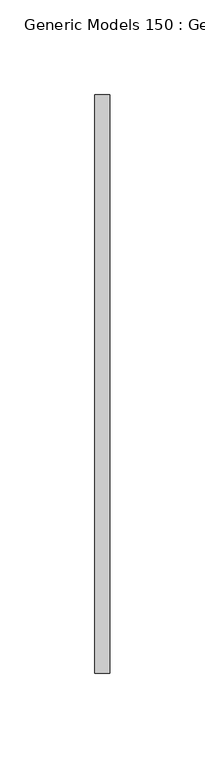
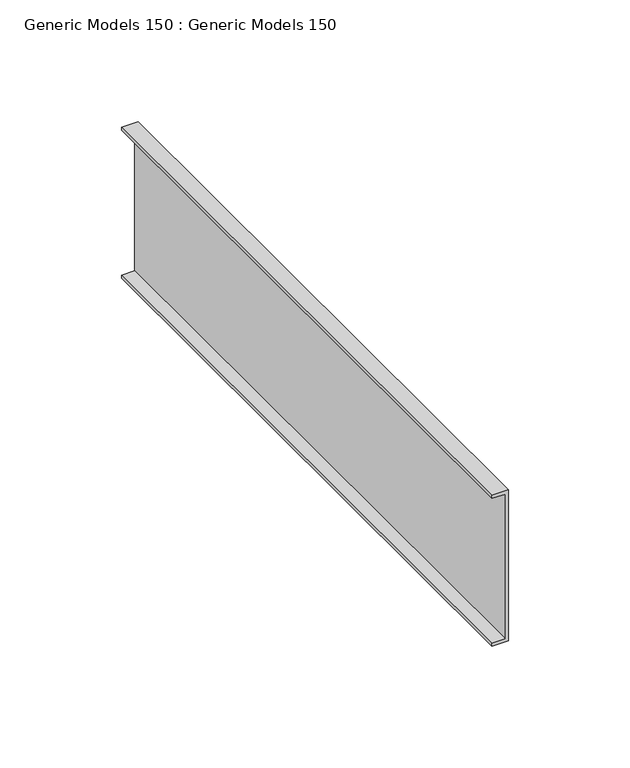
"""IFC4 building model written with IfcOpenShell, lengths in millimetres: proxy geometry, Generic Models 150 : Generic Models 150."""

from ifc_helpers import new_model, si_unit, frame, origin, place, context, project, spatial, polyline, outline, extrude, source, transform, mapped, element, save


def generic_models_150_generic_models_150_55fdb401(model_context):
    return source(origin(), model_context, "Body", "SweptSolid", [
        extrude(outline(polyline([(126267.7473366, 4973.2035579), (126195.0485482, 4973.2035579), (126195.0485482, 4966.8535579), (126193.4610482, 4966.8535579), (126193.4610482, 4974.7910579), (126269.3348366, 4974.7910579), (126269.3348366, 4966.8535579), (126267.7473366, 4966.8535579), (126267.7473366, 4973.2035579)])), frame((0.0, 399.7309662, 0.0), z_axis=(0.0, 1.0, 0.0), x_axis=(0.0, 0.0, 1.0)), (0.0, 0.0, 1.0), 304.8),
    ])


if __name__ == "__main__":
    model = new_model("IFC4")
    model_context = context("Model", 3, world=origin())
    ifc_project = project(units=[si_unit("LENGTHUNIT", "METRE", prefix="MILLI")], contexts=[model_context])
    site = spatial("IfcSite", under=ifc_project)
    building = spatial("IfcBuilding", under=site)
    placement = place(None, origin())
    generic_models_150_generic_models_150_shape = generic_models_150_generic_models_150_55fdb401(model_context)
    element("IfcBuildingElementProxy", 1, Name="Generic Models 150 : Generic Models 150", ObjectType="Generic Models 150 : Generic Models 150", at=placement, inside=building, context=model_context, shape_type="MappedRepresentation", body=[
        mapped(generic_models_150_generic_models_150_shape, transform((0.0, 0.0, 0.0), x_axis=(1.0, 0.0, 0.0), y_axis=(0.0, 1.0, 0.0), z_axis=(0.0, 0.0, 1.0))),
    ])
    save(model, "model.ifc")

# Revit data of these elements
# Element 1 (IfcBuildingElementProxy, "Generic Models 150 : Generic Models 150")
#   Materials on its faces: "_ALUM. MULLION CAP BY WINDOW MANUFACTURER (COLOR T.B.D)"
# Materials
#   "_ALUM. MULLION CAP BY WINDOW MANUFACTURER (COLOR T.B.D)": class "Metal", colour RGB 199 199 199, transparency 0, Description = "Structural steel 50ksi", Cost = 0
